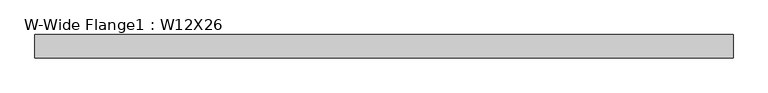
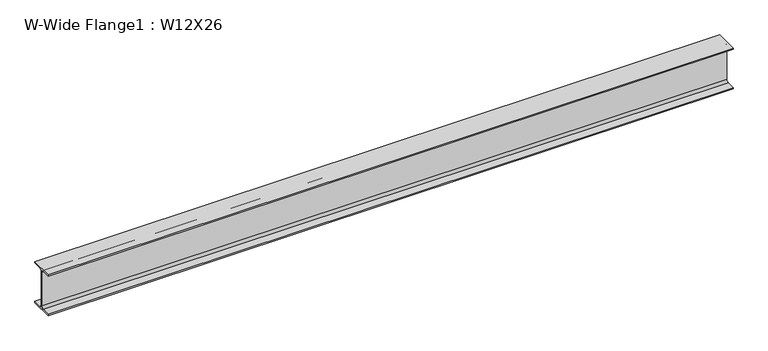
"""IFC4 building model written with IfcOpenShell, lengths in millimetres: beam geometry, W-Wide Flange1 : W12X26."""

from ifc_helpers import new_model, si_unit, point, frame, frame_2d, origin, place, context, project, spatial, polyline, circle_curve, trimmed, segment, composite_curve, outline, extrude, source, transform, mapped, element, save


def w_wide_flange1_w12x26_4e65a3b6(model_context):
    return source(origin(), model_context, "Body", "SweptSolid", [
        extrude(outline(composite_curve([segment(polyline([(82.423, -145.288), (82.423, -154.94), (-82.423, -154.94), (-82.423, -145.288), (-20.2565, -145.288)]), True, "CONTINUOUS"), segment(trimmed(circle_curve(frame_2d((-20.2565, -127.9525)), 17.3355), [point((-20.2565, -145.288))], [point((-2.921, -127.9525))], True, "CARTESIAN"), True, "CONTINUOUS"), segment(polyline([(-2.921, -127.9525), (-2.921, 127.9525)]), True, "CONTINUOUS"), segment(trimmed(circle_curve(frame_2d((-20.2565, 127.9525)), 17.3355), [point((-2.921, 127.9525))], [point((-20.2565, 145.288))], True, "CARTESIAN"), True, "CONTINUOUS"), segment(polyline([(-20.2565, 145.288), (-82.423, 145.288), (-82.423, 154.94), (82.423, 154.94), (82.423, 145.288), (20.2565, 145.288)]), True, "CONTINUOUS"), segment(trimmed(circle_curve(frame_2d((20.2565, 127.9525)), 17.3355), [point((20.2565, 145.288))], [point((2.921, 127.9525))], True, "CARTESIAN"), True, "CONTINUOUS"), segment(polyline([(2.921, 127.9525), (2.921, -127.9525)]), True, "CONTINUOUS"), segment(trimmed(circle_curve(frame_2d((20.2565, -127.9525)), 17.3355), [point((2.921, -127.9525))], [point((20.2565, -145.288))], True, "CARTESIAN"), True, "CONTINUOUS"), segment(polyline([(20.2565, -145.288), (82.423, -145.288)]), True, "CONTINUOUS")], self_intersect=False)), frame((-2456.6945104, 0.0, 0.0), z_axis=(1.0, 0.0, 0.0), x_axis=(0.0, 1.0, 0.0)), (0.0, 0.0, 1.0), 4916.1316964),
    ])


if __name__ == "__main__":
    model = new_model("IFC4")
    model_context = context("Model", 3, world=origin())
    ifc_project = project(units=[si_unit("LENGTHUNIT", "METRE", prefix="MILLI")], contexts=[model_context])
    site = spatial("IfcSite", under=ifc_project)
    building = spatial("IfcBuilding", under=site)
    placement = place(None, origin())
    w_wide_flange1_w12x26_shape = w_wide_flange1_w12x26_4e65a3b6(model_context)
    element("IfcBeam", 1, ObjectType="W-Wide Flange1 : W12X26", at=placement, inside=building, context=model_context, shape_type="MappedRepresentation", body=[
        mapped(w_wide_flange1_w12x26_shape, transform((0.0, 0.0, 0.0), x_axis=(1.0, 0.0, 0.0), y_axis=(0.0, 1.0, 0.0), z_axis=(0.0, 0.0, 1.0))),
    ])
    save(model, "model.ifc")

# Revit data of these elements
# Type "W-Wide Flange1 : W12X26"
#   Assembly Code = "B10"
#   W = 26
#   Start Extension Calculation [instance default] = 10' - 0"
#   Start Extension [instance default] = -0' - 0 1/2"
#   End Extension Calculation [instance default] = 10' - 0"
#   End Extension [instance default] = -0' - 0 1/2"
#   Length [instance default] = 5' - 0"
#   bf = 0' - 6.49"
#   d = 1' - 0.2"
#   k = 0' - 1 1/16"
#   k2 = 0' - 0.6825"
#   tf = 0' - 0.38"
#   tw = 0' - 0.23"
#   A = 0.053125 SF
#   Structural Material [instance default] = Metal - Steel - ASTM A992
# Element 1 (IfcBeam, "W-Wide Flange1 : W12X26")
#   Materials on its faces: "Metal - Steel - ASTM A992"
# Materials
#   "Metal - Steel - ASTM A992": class "Metal", colour RGB 199 199 199, transparency 0
